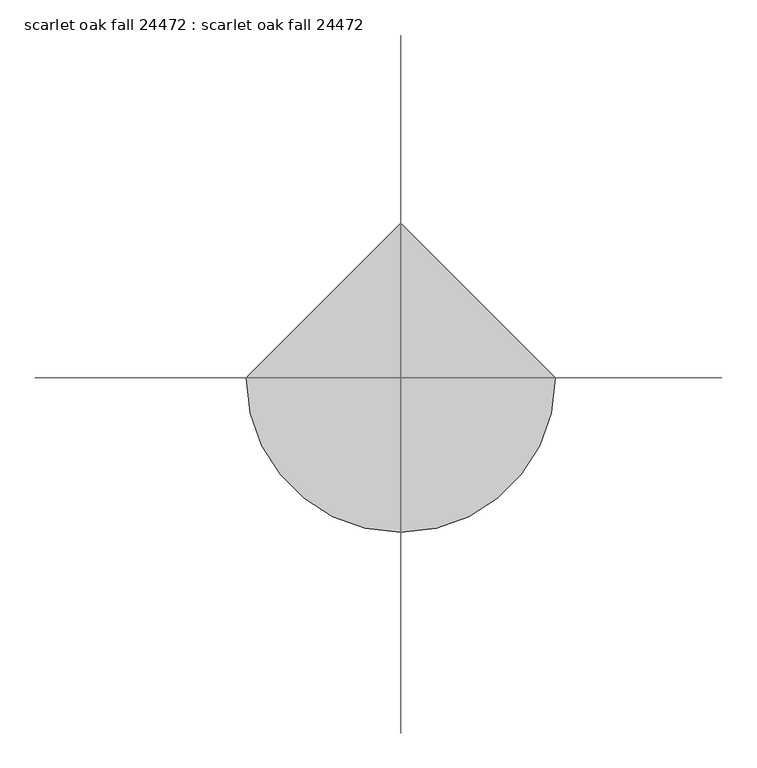
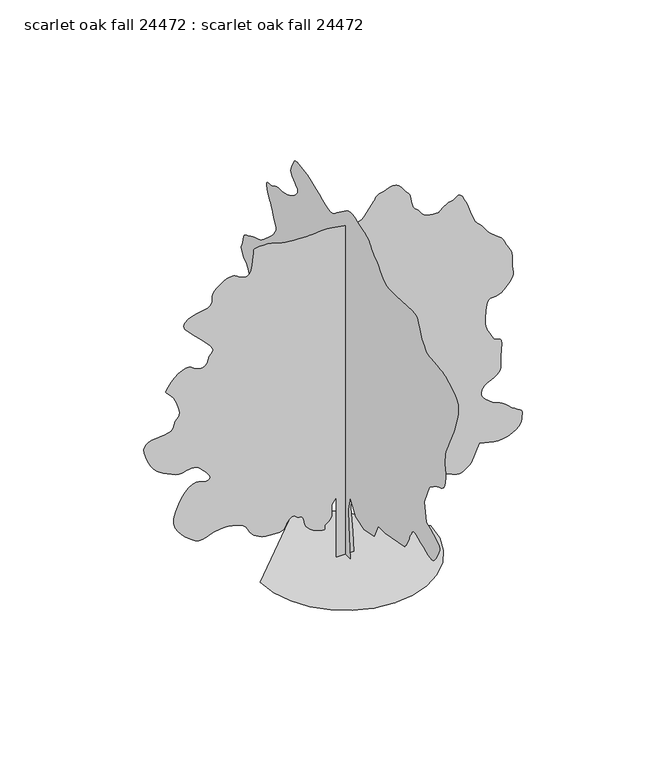
"""IFC4 building model written with IfcOpenShell, lengths in millimetres: proxy geometry, scarlet oak fall 24472 : scarlet oak fall 24472."""

import ifcopenshell
import ifcopenshell.guid

model = None  # the IFC model being written
_history = None  # IfcOwnerHistory: only IFC2X3 demands one
_inside = {}  # id of a spatial element -> (the spatial element, [elements in it])
_under = {}  # id of a project, library or spatial element -> (it, [spatial elements below it])
_declared = {}  # id of a project -> (the project, [libraries it declares])
_typed = {}  # id of a type object -> (the type object, [elements of that type])
_made_of = {}  # id of a material, layer set ... -> (it, [elements and type objects made of it])


def new_model(schema):
    """Start an empty IFC model of exactly this schema.

    Asked for "IFC4X3", IfcOpenShell would pick the latest addendum, in which some entities
    have other attributes; the version numbers below select the first issue.
    IFC2X3 requires an IfcOwnerHistory on every rooted entity: one is made here for all.
    """
    global model, _history
    if schema == "IFC4X3":
        model = ifcopenshell.file(schema_version=(4, 3, 0, 0))
    else:
        model = ifcopenshell.file(schema=schema)
    _inside.clear()
    _under.clear()
    _declared.clear()
    _typed.clear()
    _made_of.clear()
    _history = None
    if model.schema == "IFC2X3":
        org = make("IfcOrganization", Name="unknown")
        user = make(
            "IfcPersonAndOrganization",
            ThePerson=make("IfcPerson", FamilyName="unknown"),
            TheOrganization=org,
        )
        app = make(
            "IfcApplication",
            ApplicationDeveloper=org,
            Version="unknown",
            ApplicationFullName="unknown",
            ApplicationIdentifier="unknown",
        )
        _history = make(
            "IfcOwnerHistory",
            OwningUser=user,
            OwningApplication=app,
            ChangeAction="ADDED",
            CreationDate=0,
        )
    return model


def make(cls, **values):
    """One entity of the class cls with the attributes given. An attribute that is None is left unset."""
    return model.create_entity(
        cls, **{name: value for name, value in values.items() if value is not None}
    )


def rooted(cls, **values):
    """An entity with a GlobalId (a new one), such as an element, a storey or a relation."""
    return make(cls, GlobalId=ifcopenshell.guid.new(), OwnerHistory=_history, **values)


def si_unit(unit_type, name, prefix=None):
    """IfcSIUnit, for example si_unit("LENGTHUNIT", "METRE", prefix="MILLI")."""
    return make("IfcSIUnit", UnitType=unit_type, Prefix=prefix, Name=name)


def assignment(units):
    """IfcUnitAssignment: the units of a project."""
    return None if units is None else make("IfcUnitAssignment", Units=units)


def point(xyz):
    """IfcCartesianPoint."""
    return None if xyz is None else make("IfcCartesianPoint", Coordinates=xyz)


def direction(xyz):
    """IfcDirection."""
    return None if xyz is None else make("IfcDirection", DirectionRatios=xyz)


def frame(location, z_axis=None, x_axis=None):
    """IfcAxis2Placement3D, a coordinate frame: its origin and axes. An axis left out is left unset."""
    return make(
        "IfcAxis2Placement3D",
        Location=point(location),
        Axis=direction(z_axis),
        RefDirection=direction(x_axis),
    )


def origin():
    """The frame at (0, 0, 0) with its axes left unset."""
    return frame((0.0, 0.0, 0.0))


def place(relative_to, where):
    """IfcLocalPlacement: puts the frame where relative to a parent placement (None: the world)."""
    return make(
        "IfcLocalPlacement", PlacementRelTo=relative_to, RelativePlacement=where
    )


def context(
    kind, dimensions, precision=None, world=None, true_north=None, identifier=None
):
    """IfcGeometricRepresentationContext, for example the 3D "Model" context."""
    return make(
        "IfcGeometricRepresentationContext",
        ContextIdentifier=identifier,
        ContextType=kind,
        CoordinateSpaceDimension=dimensions,
        Precision=precision,
        WorldCoordinateSystem=world,
        TrueNorth=true_north,
    )


def project(units=None, contexts=None):
    """IfcProject with its units and contexts."""
    return rooted(
        "IfcProject",
        Name="project",
        RepresentationContexts=contexts,
        UnitsInContext=assignment(units),
    )


def spatial(cls, under=None, at=None, **own):
    """A site, building, storey or space (cls), placed at a placement, below another one or the project."""
    s = rooted(cls, ObjectPlacement=at, **own)
    if under is not None:
        _under.setdefault(under.id(), (under, []))[1].append(s)
    return s


def point_list(points):
    """IfcCartesianPointList2D or 3D."""
    cls = (
        "IfcCartesianPointList2D" if len(points[0]) == 2 else "IfcCartesianPointList3D"
    )
    return make(cls, CoordList=points)


def triangles(points, corners, closed=None, point_numbers=None):
    """IfcTriangulatedFaceSet: each triangle names its three corners, points numbered from 1."""
    return make(
        "IfcTriangulatedFaceSet",
        Coordinates=point_list(points),
        Closed=closed,
        CoordIndex=corners,
        PnIndex=point_numbers,
    )


def shape(context_of_items, identifier, shape_type, items):
    """IfcShapeRepresentation: the items that make up one representation, for example the "Body"."""
    return make(
        "IfcShapeRepresentation",
        ContextOfItems=context_of_items,
        RepresentationIdentifier=identifier,
        RepresentationType=shape_type,
        Items=items,
    )


def source(mapping_origin, context_of_items, identifier, shape_type, items):
    """IfcRepresentationMap: a shape defined once, which mapped items show again and again."""
    return make(
        "IfcRepresentationMap",
        MappingOrigin=mapping_origin,
        MappedRepresentation=shape(context_of_items, identifier, shape_type, items),
    )


def transform(
    local_origin,
    x_axis=None,
    y_axis=None,
    z_axis=None,
    scale=None,
    scale2=None,
    scale3=None,
    uniform=True,
):
    """IfcCartesianTransformationOperator3D, or its non-uniform kind. x_axis, y_axis, z_axis: its Axis1, 2, 3."""
    if uniform:
        return make(
            "IfcCartesianTransformationOperator3D",
            Axis1=direction(x_axis),
            Axis2=direction(y_axis),
            LocalOrigin=point(local_origin),
            Scale=scale,
            Axis3=direction(z_axis),
        )
    return make(
        "IfcCartesianTransformationOperator3DnonUniform",
        Axis1=direction(x_axis),
        Axis2=direction(y_axis),
        LocalOrigin=point(local_origin),
        Scale=scale,
        Axis3=direction(z_axis),
        Scale2=scale2,
        Scale3=scale3,
    )


def mapped(mapping_source, mapping_target):
    """IfcMappedItem: shows the shape of a source again, moved by a transform."""
    return make(
        "IfcMappedItem", MappingSource=mapping_source, MappingTarget=mapping_target
    )


def made_of(thing, what):
    """Note that an element or type object is made of a material, layer set ...; save() writes the relation."""
    if what is not None:
        _made_of.setdefault(what.id(), (what, []))[1].append(thing)
    return thing


def element(
    cls,
    number,
    at=None,
    inside=None,
    cuts=None,
    type_object=None,
    material=None,
    context=None,
    identifier="Body",
    shape_type=None,
    held_by="IfcProductDefinitionShape",
    body=None,
    shapes=None,
    **own,
):
    """One element of the class cls, such as IfcWall. Its Tag is "e" and its number.

    at: its placement. inside: the storey or other place that contains it. cuts: it is an
    opening in that element (IfcRelVoidsElement). A single representation is given by context,
    identifier, shape_type and body (its items); several are given by shapes. held_by: the class
    of the entity that holds the representations. save() writes the other relations.
    """
    e = rooted(cls, Tag="e%d" % number, ObjectPlacement=at, **own)
    if body is not None:
        shapes = [shape(context, identifier, shape_type, body)]
    if shapes is not None:
        e.Representation = make(held_by, Representations=shapes)
    if inside is not None:
        _inside.setdefault(inside.id(), (inside, []))[1].append(e)
    if cuts is not None:
        rooted(
            "IfcRelVoidsElement", RelatingBuildingElement=cuts, RelatedOpeningElement=e
        )
    if type_object is not None:
        _typed.setdefault(type_object.id(), (type_object, []))[1].append(e)
    return made_of(e, material)


def aggregate(whole, parts):
    """IfcRelAggregates: a whole, such as a stair, and the parts it consists of."""
    return rooted("IfcRelAggregates", RelatingObject=whole, RelatedObjects=parts)


def save(model, path):
    """Write the relations noted so far, then the file.

    IfcRelAggregates (storeys below a building ...), IfcRelContainedInSpatialStructure (elements
    in a storey), IfcRelDefinesByType, IfcRelAssociatesMaterial and IfcRelDeclares: one each for
    every whole, place, type object, material and project.
    """
    for whole, parts in _under.values():
        aggregate(whole, parts)
    for where, things in _inside.values():
        rooted(
            "IfcRelContainedInSpatialStructure",
            RelatedElements=things,
            RelatingStructure=where,
        )
    for kind, things in _typed.values():
        rooted("IfcRelDefinesByType", RelatedObjects=things, RelatingType=kind)
    for what, things in _made_of.values():
        rooted("IfcRelAssociatesMaterial", RelatedObjects=things, RelatingMaterial=what)
    for by, libraries in _declared.values():
        rooted("IfcRelDeclares", RelatingContext=by, RelatedDefinitions=libraries)
    model.write(path)


def scarlet_oak_fall_24472_scarlet_oak_fall_24472_7ddbc09d(model_context):
    return source(origin(), model_context, "Body", "Tessellation", [
        triangles([(0.0175265, 310.9036245, 0.0), (0.0175265, -298.2620451, 0.0), (0.0175265, -200.0097575, 1159.3779247), (0.0175265, -180.3587949, 1709.5902706), (0.0175265, -298.2620451, 2220.5035618), (0.0175265, -612.6708881, 1709.5902706), (0.0175265, -1123.5817085, 1552.3870754), (0.0175265, -1713.0954346, 1689.9407433), (0.0175265, -1948.9013901, 2181.2021816), (0.0175265, -2361.5625389, 2181.2021816), (0.0175265, -3501.2886108, 2397.3587551), (0.0175265, -3543.2238419, 2447.9453476), (0.0175265, -3584.1434372, 2498.8747971), (0.0175265, -3622.9800201, 2550.4902512), (0.0175265, -3658.7176643, 2603.1445953), (0.0175265, -3690.3407341, 2657.1703674), (0.0175265, -3716.8074326, 2712.9233597), (0.0175265, -3737.102124, 2770.7082047), (0.0175265, -3756.8125488, 2830.2458496), (0.0175265, -3781.6790543, 2890.7994209), (0.0175265, -3810.8383209, 2952.2166023), (0.0175265, -3843.4264481, 3014.3197884), (0.0175265, -3878.6054054, 3076.9307922), (0.0175265, -3915.4862938, 3139.8972977), (0.0175265, -3953.2560814, 3203.0164101), (0.0175265, -3971.239286, 3223.4125488), (0.0175265, -3996.1057915, 3239.8717186), (0.0175265, -4034.7139, 3248.4060814), (0.0175265, -4093.9466217, 3245.0786682), (0.0175265, -4180.6878387, 3225.9525101), (0.0175265, -4301.7949814, 3187.039769), (0.0175265, -4464.1516411, 3124.4287651), (0.0175265, -4635.5763519, 3050.7434372), (0.0175265, -4781.5502907, 2984.9826256), (0.0175265, -4905.5273163, 2932.6079155), (0.0175265, -5010.9377426, 2899.1561783), (0.0175265, -5101.2345566, 2890.113707), (0.0175265, -5179.8222015, 2910.9670853), (0.0175265, -5250.1801163, 2967.228186), (0.0175265, -5321.172876, 3055.8486488), (0.0175265, -5394.553862, 3163.7225876), (0.0175265, -5463.1339783, 3281.2229736), (0.0175265, -5519.6741318, 3398.7233597), (0.0175265, -5556.9613907, 3506.5970078), (0.0175265, -5567.8072403, 3595.2430504), (0.0175265, -5544.9470078, 3654.9838806), (0.0175265, -5489.0922775, 3699.9671814), (0.0175265, -5408.4727798, 3750.0815643), (0.0175265, -5307.2539581, 3804.513707), (0.0175265, -5189.4995178, 3862.3750008), (0.0175265, -5059.4004822, 3922.8268341), (0.0175265, -4921.0467178, 3984.9805984), (0.0175265, -4778.5783791, 4047.9982635), (0.0175265, -4660.6716225, 4716.1196915), (0.0175265, -4955.4132248, 5403.875386), (0.0175265, -4964.7097504, 5417.0071426), (0.0175265, -4979.1367767, 5433.0346527), (0.0175265, -5003.9015442, 5454.9298279), (0.0175265, -5044.1101364, 5485.5872589), (0.0175265, -5104.9430511, 5527.903862), (0.0175265, -5191.5825302, 5584.850386), (0.0175265, -5309.1334946, 5659.3487457), (0.0175265, -5436.6669891, 5726.8364868), (0.0175265, -5549.7478775, 5770.9308884), (0.0175265, -5648.4011581, 5806.7955597), (0.0175265, -5732.6279938, 5849.5441132), (0.0175265, -5802.4016418, 5914.2884171), (0.0175265, -5857.7482635, 6016.1426651), (0.0175265, -5898.6422791, 6170.2443054), (0.0175265, -5922.3152527, 6321.6030899), (0.0175265, -5929.1223953, 6418.6564682), (0.0175265, -5923.915155, 6481.6735519), (0.0175265, -5911.4694031, 6530.949614), (0.0175265, -5896.6354248, 6586.7537659), (0.0175265, -5884.2152527, 6669.354538), (0.0175265, -5879.0080124, 6799.0722015), (0.0175265, -5880.8369705, 6942.175676), (0.0175265, -5888.8632248, 7060.8701752), (0.0175265, -5906.8464294, 7169.2769302), (0.0175265, -5938.5712372, 7281.4433395), (0.0175265, -5987.8467178, 7411.4917969), (0.0175265, -6058.4336884, 7573.5179535), (0.0175265, -6154.0900589, 7781.5947876), (0.0175265, -6244.9205612, 7969.6821442), (0.0175265, -6305.4738419, 8083.1694031), (0.0175265, -6346.419017, 8153.3494217), (0.0175265, -6378.4484573, 8211.4900589), (0.0175265, -6412.2045364, 8288.8835907), (0.0175265, -6458.3057922, 8416.8234558), (0.0175265, -6527.4701752, 8626.5513519), (0.0175265, -6601.9935333, 8869.1720078), (0.0175265, -6652.1329147, 9078.1127426), (0.0175265, -6670.2940155, 9258.1732635), (0.0175265, -6648.9075302, 9414.1800201), (0.0175265, -6580.4541504, 9550.9338821), (0.0175265, -6457.3407349, 9673.2345566), (0.0175265, -6271.9968155, 9785.9340729), (0.0175265, -6092.164769, 9878.5679535), (0.0175265, -5973.8772217, 9942.3477814), (0.0175265, -5892.0130325, 9984.43591), (0.0175265, -5821.4772217, 10012.1214294), (0.0175265, -5737.1998077, 10032.5690186), (0.0175265, -5614.0858109, 10053.0154449), (0.0175265, -5427.0402512, 10080.7009644), (0.0175265, -5226.405986, 10102.5205627), (0.0175265, -5070.8056, 10110.9526062), (0.0175265, -4947.513707, 10121.4182465), (0.0175265, -4843.8310822, 10149.4339783), (0.0175265, -4747.0061783, 10210.4442078), (0.0175265, -4644.3394798, 10319.9445007), (0.0175265, -4523.1050194, 10493.3501953), (0.0175265, -4417.2379349, 10684.0025116), (0.0175265, -4354.6778, 10837.2152527), (0.0175265, -4313.7837845, 10956.3661194), (0.0175265, -4272.8641891, 11044.9362946), (0.0175265, -4210.3040543, 11106.353476), (0.0175265, -4104.4369698, 11144.0476868), (0.0175265, -3933.5965256, 11161.4710419), (0.0175265, -2990.3674713, 11102.5176636), (0.0175265, -2816.5045372, 11105.5663147), (0.0175265, -2674.9503868, 11105.1593628), (0.0175265, -2554.6812744, 11112.322879), (0.0175265, -2444.7449615, 11138.027124), (0.0175265, -2334.1178478, 11193.3225861), (0.0175265, -2211.8040928, 11289.1574341), (0.0175265, -2066.8032051, 11436.5786682), (0.0175265, -1927.0752514, 11585.474231), (0.0175265, -1822.4043148, 11686.9215271), (0.0175265, -1744.5483112, 11753.6721039), (0.0175265, -1685.2519306, 11798.4275116), (0.0175265, -1636.2706181, 11833.8858124), (0.0175265, -1589.3492088, 11872.7729736), (0.0175265, -1536.2428574, 11927.8405426), (0.0175265, -1485.2548359, 11992.8644806), (0.0175265, -1443.5456085, 12053.4177612), (0.0175265, -1401.1529926, 12109.8573395), (0.0175265, -1348.1024517, 12162.4855225), (0.0175265, -1274.4272976, 12211.7104248), (0.0175265, -1170.1577173, 12257.8366791), (0.0175265, -1025.3294209, 12301.1944977), (0.0175265, -862.7415253, 12348.971814), (0.0175265, -711.1517956, 12401.9057922), (0.0175265, -569.5289721, 12450.7249054), (0.0175265, -436.8469909, 12486.1320465), (0.0175265, -312.0695054, 12498.8580139), (0.0175265, -194.1657283, 12479.604538), (0.0175265, -82.1065163, 12419.1012543), (0.0175265, 507.4081999, 11986.7939209), (0.0175265, 571.2282506, 11928.7044434), (0.0175265, 632.9883253, 11875.7704651), (0.0175265, 700.2449759, 11833.124231), (0.0175265, 780.5673986, 11805.9712372), (0.0175265, 881.5121092, 11799.4437286), (0.0175265, 1010.6431807, 11818.6960419), (0.0175265, 1175.5247589, 11868.8871643), (0.0175265, 1362.6338322, 11943.4105225), (0.0175265, 1551.1170948, 12027.2309875), (0.0175265, 1737.537838, 12112.7780914), (0.0175265, 1918.4594982, 12192.4581116), (0.0175265, 2090.445512, 12258.7517395), (0.0175265, 2250.0539383, 12304.0652527), (0.0175265, 2393.8535912, 12320.8549255), (0.0175265, 2524.6458984, 12330.0241333), (0.0175265, 2646.1466217, 12350.8775116), (0.0175265, 2756.3317566, 12373.4331116), (0.0175265, 2853.0805023, 12387.7578186), (0.0175265, 2934.3860046, 12383.8720093), (0.0175265, 2998.139962, 12351.7914093), (0.0175265, 3042.3105217, 12281.5352325), (0.0175265, 3081.7819496, 12193.2708527), (0.0175265, 3127.0957535, 12111.863031), (0.0175265, 3169.6661201, 12034.5712372), (0.0175265, 3200.9081085, 11958.6502899), (0.0175265, 3212.1856178, 11881.3840759), (0.0175265, 3194.9389961, 11799.9762543), (0.0175265, 3140.5830116, 11711.6862946), (0.0175265, 3057.3979729, 11630.7877441), (0.0175265, 2968.3455597, 11567.4148682), (0.0175265, 2886.8880318, 11512.6519318), (0.0175265, 2826.3850388, 11457.5343658), (0.0175265, 2800.2738419, 11393.1452728), (0.0175265, 2821.9146721, 11310.5445007), (0.0175265, 2904.7694984, 11200.765155), (0.0175265, 3019.1712364, 11091.3927612), (0.0175265, 3127.0448845, 11011.6115845), (0.0175265, 3229.076738, 10954.8173767), (0.0175265, 3325.9522202, 10914.5582062), (0.0175265, 3418.3576263, 10884.2309875), (0.0175265, 3507.0033783, 10857.3826263), (0.0175265, 3592.525193, 10827.4112), (0.0175265, 3677.9455605, 10804.3219116), (0.0175265, 3765.7785713, 10796.7026093), (0.0175265, 3855.9995178, 10795.9654449), (0.0175265, 3948.6333984, 10793.5016418), (0.0175265, 4043.6802132, 10780.7256775), (0.0175265, 4141.139962, 10749.0264496), (0.0175265, 4240.9873558, 10689.8695953), (0.0175265, 4344.1874519, 10637.3169891), (0.0175265, 4445.6350388, 10618.4704651), (0.0175265, 4536.4402519, 10614.0509674), (0.0175265, 4607.6617767, 10604.8306), (0.0175265, 4650.3338814, 10571.5570496), (0.0175265, 4655.540831, 10494.9500977), (0.0175265, 4614.3674721, 10355.8085907), (0.0175265, 4553.5089775, 10209.3779938), (0.0175265, 4502.988224, 10110.7247131), (0.0175265, 4458.6400589, 10040.2394806), (0.0175265, 4416.3743248, 9978.3653503), (0.0175265, 4372.025869, 9905.4918915), (0.0175265, 4321.4798264, 9802.0377411), (0.0175265, 4260.6469116, 9648.393631), (0.0175265, 4196.3595566, 9497.2633209), (0.0175265, 4141.038224, 9401.8104263), (0.0175265, 4098.7472008, 9343.1361008), (0.0175265, 4073.6522209, 9302.3438232), (0.0175265, 4069.8675682, 9260.5353287), (0.0175265, 4091.5336876, 9198.7629364), (0.0175265, 4142.740155, 9098.1789597), (0.0175265, 4233.9008698, 8964.8539581), (0.0175265, 4361.815155, 8823.2998077), (0.0175265, 4510.3796333, 8682.0758698), (0.0175265, 4663.3894798, 8549.7926651), (0.0175265, 4804.7404449, 8435.0357162), (0.0175265, 4918.2277039, 8346.4149628), (0.0175265, 4987.7217178, 8292.4909286), (0.0175265, 5049.4185333, 8258.7592667), (0.0175265, 5142.0524139, 8224.6723938), (0.0175265, 5253.2537659, 8189.9000977), (0.0175265, 5370.6524139, 8154.0860046), (0.0175265, 5481.8537659, 8116.9004837), (0.0175265, 5574.4876465, 8078.0133224), (0.0175265, 5636.1838806, 8037.0425674), (0.0175265, 5687.8475876, 8003.0068542), (0.0175265, 5753.6336884, 7978.9530899), (0.0175265, 5825.9217178, 7955.5853302), (0.0175265, 5897.1941116, 7923.6064682), (0.0175265, 5959.8815643, 7873.7717194), (0.0175265, 6006.3891907, 7796.7589783), (0.0175265, 6029.1982635, 7683.3222977), (0.0175265, 6047.8674728, 7569.3780899), (0.0175265, 6079.9474915, 7488.7835907), (0.0175265, 6114.7709473, 7429.1447891), (0.0175265, 6141.7204651, 7378.0903473), (0.0175265, 6150.0769318, 7323.2774139), (0.0175265, 6129.2235535, 7252.2846542), (0.0175265, 6068.4917953, 7152.7674728), (0.0175265, 5993.1045364, 7059.5493256), (0.0175265, 5932.1448853, 7003.8213318), (0.0175265, 5880.8113907, 6967.6776077), (0.0175265, 5834.2787659, 6933.2349426), (0.0175265, 5787.7711395, 6882.638031), (0.0175265, 5736.437645, 6798.030986), (0.0175265, 5675.4779938, 6661.5055984), (0.0175265, 5609.0314682, 6524.7523178), (0.0175265, 5548.0712357, 6438.5447891), (0.0175265, 5498.1097504, 6383.604538), (0.0175265, 5464.6577225, 6340.6786697), (0.0175265, 5453.2026077, 6290.5642868), (0.0175265, 5469.2295364, 6213.9579163), (0.0175265, 5518.277124, 6091.6566605), (0.0175265, 5583.4283798, 5957.8747101), (0.0175265, 5644.7694031, 5854.0141891), (0.0175265, 5703.392569, 5771.4645767), (0.0175265, 5760.2629349, 5701.6141891), (0.0175265, 5816.4734573, 5635.9048279), (0.0175265, 5873.0136108, 5565.7242279), (0.0175265, 5930.9257736, 5482.4886108), (0.0175265, 5998.1338806, 5400.3959473), (0.0175265, 6076.3407349, 5333.4157333), (0.0175265, 6157.2904449, 5272.6339783), (0.0175265, 6232.753862, 5209.0832062), (0.0175265, 6294.4506775, 5133.8738434), (0.0175265, 6334.1505798, 5038.0139969), (0.0175265, 6343.5994217, 4912.614093), (0.0175265, 6351.5495178, 4814.1384178), (0.0175265, 6380.8355209, 4781.651738), (0.0175265, 6414.2369705, 4780.1024139), (0.0175265, 6434.5822403, 4774.4382248), (0.0175265, 6424.6508698, 4729.5816605), (0.0175265, 6367.3229736, 4610.4810814), (0.0175265, 6245.3519302, 4382.0589775), (0.0175265, 6117.819017, 4125.8490349), (0.0175265, 6040.8312744, 3937.3811783), (0.0175265, 5992.6981659, 3802.5071434), (0.0175265, 5951.8041504, 3707.1809853), (0.0175265, 5896.4575287, 3637.2800194), (0.0175265, 5805.0177612, 3578.7330116), (0.0175265, 5655.8437271, 3517.4428574), (0.0175265, 5483.6059845, 3467.7098465), (0.0175265, 5332.0187256, 3446.8561775), (0.0175265, 5192.8016418, 3445.2559845), (0.0175265, 5057.7244217, 3453.2825294), (0.0175265, 4918.5067566, 3461.2834946), (0.0175265, 4766.9197884, 3459.6833015), (0.0175265, 4594.7076256, 3438.8299232), (0.0175265, 4422.952993, 3420.1610046), (0.0175265, 4274.5661201, 3424.1741318), (0.0175265, 4144.0610046, 3439.8714294), (0.0175265, 4025.9254829, 3456.2544411), (0.0175265, 3914.6735527, 3462.3250008), (0.0175265, 3804.7930504, 3447.0849426), (0.0175265, 3690.7723938, 3399.5361008), (0.0175265, 3581.6540543, 3348.9900581), (0.0175265, 3491.4078186, 3322.5233597), (0.0175265, 3422.1419884, 3305.6831085), (0.0175265, 3375.9139961, 3284.0422783), (0.0175265, 3354.7812744, 3243.1229736), (0.0175265, 3360.8009651, 3168.5484558), (0.0175265, 3396.0307915, 3045.815831), (0.0175265, 3452.8505791, 2915.4374519), (0.0175265, 3521.0243248, 2823.1846527), (0.0175265, 3598.6722015, 2762.7581085), (0.0175265, 3683.8638039, 2727.7567566), (0.0175265, 3774.7195953, 2711.8309845), (0.0175265, 3869.3600395, 2708.6053093), (0.0175265, 3965.8800201, 2711.7548264), (0.0175265, 4339.2598457, 2299.1064674), (0.0175265, 4368.5208504, 2252.6422977), (0.0175265, 4396.5877419, 2205.3220757), (0.0175265, 4422.2672791, 2156.2823364), (0.0175265, 4444.3144798, 2104.6617954), (0.0175265, 4461.5608109, 2049.6073071), (0.0175265, 4472.7877419, 1990.2551159), (0.0175265, 4476.800869, 1925.7468441), (0.0175265, 4476.115155, 1858.4875774), (0.0175265, 4471.314576, 1791.9167862), (0.0175265, 4458.2333977, 1726.7225098), (0.0175265, 4432.8082054, 1663.588282), (0.0175265, 4390.8726837, 1603.2049038), (0.0175265, 4328.3125488, 1546.2580891), (0.0175265, 4240.9873558, 1493.4361679), (0.0175265, 4157.7008698, 1448.5772781), (0.0175265, 4099.153862, 1413.687838), (0.0175265, 4049.1917953, 1386.7054733), (0.0175265, 3991.6610046, 1365.5650486), (0.0175265, 3910.4316605, 1348.2066605), (0.0175265, 3789.3245178, 1332.5653187), (0.0175265, 3612.1850395, 1316.5811199), (0.0175265, 3410.6865829, 1318.8721138), (0.0175265, 3225.0127419, 1354.1629829), (0.0175265, 3051.7084946, 1414.5488319), (0.0175265, 2887.3449806, 1492.1179344), (0.0175265, 2728.4933395, 1578.9707726), (0.0175265, 2571.6738419, 1667.1976547), (0.0175265, 2413.5029732, 1748.8916508), (0.0175265, 2272.4543152, 1823.1968536), (0.0175265, 2163.3739094, 1893.3770176), (0.0175265, 2077.3237839, 1957.7152416), (0.0175265, 2005.3681469, 2014.4892471), (0.0175265, 1938.5687359, 2061.9822784), (0.0175265, 1867.9871429, 2098.4769985), (0.0175265, 1784.687867, 2122.2512741), (0.0175265, 1693.0802319, 2142.3020851), (0.0175265, 1602.8492569, 2167.1661198), (0.0175265, 1512.9611389, 2194.438147), (0.0175265, 1422.387307, 2221.7075581), (0.0175265, 1330.0913418, 2246.5715927), (0.0175265, 1235.0471432, 2266.6224037), (0.0175265, 1136.2233061, 2279.4544693), (0.0175265, 1035.1643583, 2286.1575485), (0.0175265, 934.1027945, 2289.7669212), (0.0175265, 833.0438467, 2290.7981083), (0.0175265, 731.9848263, 2289.7669212), (0.0175265, 630.9258785, 2287.1887356), (0.0175265, 529.864351, 2283.5795082), (0.0175265, 428.8053669, 2279.4544693), (0.0175265, 232.3013002, 1984.6976063), (0.0175265, 192.9998656, 1532.7376934), (284.9321357, 0.0006104, 0.0093596), (-304.5815722, 0.0006104, 0.0093596), (-304.5815722, 0.0004832, 2161.5603573), (-461.7872563, 0.0004832, 1945.4063999), (-461.7872563, 0.0005087, 1709.6004444), (-458.17792, 0.0005087, 1654.888813), (-458.17792, 0.0005087, 1600.3473747), (-465.3965927, 0.0005087, 1546.1514095), (-483.4407675, 0.0005341, 1492.4709652), (-515.9248312, 0.0005341, 1439.4789963), (-566.4555768, 0.0005341, 1387.3429344), (-638.6398699, 0.0005341, 1336.2406757), (-695.1853283, 0.0005341, 1283.1902802), (-710.8266701, 0.0005341, 1229.4514091), (-707.2172974, 0.0005341, 1181.559783), (-706.0133738, 0.0005341, 1146.037896), (-728.8733156, 0.0005341, 1129.4237211), (-797.4482723, 0.0005341, 1138.2476738), (-933.3966602, 0.0005341, 1179.0375532), (-1088.4814528, 0.0005341, 1242.5731373), (-1204.3791023, 0.0005341, 1314.3561104), (-1287.6199516, 0.0005341, 1393.0172974), (-1344.7395756, 0.0005341, 1477.1750965), (-1382.2654827, 0.0005087, 1565.4579346), (-1406.7282337, 0.0005087, 1656.4914768), (-1424.6607147, 0.0005087, 1748.9018246), (-1429.2428478, 0.0005087, 1774.0502895), (-1436.0601643, 0.0005087, 1798.5130405), (-1447.3453766, 0.0005087, 1821.6042183), (-1465.3361389, 0.0005087, 1842.6277897), (-1492.2602222, 0.0005087, 1860.9031277), (-1530.3602222, 0.0005087, 1875.7417568), (-1581.8637646, 0.0005087, 1886.4554924), (-1633.3673069, 0.0005087, 1904.0983109), (-1673.8702126, 0.0005087, 1933.7757145), (-1709.219363, 0.0004832, 1965.8584946), (-1745.2543728, 0.0004832, 1990.7225292), (-1787.8222687, 0.0004832, 1998.7438419), (-1842.7623745, 0.0004832, 1980.2958401), (-1915.9220078, 0.0005087, 1925.7544018), (-1980.257761, 0.0005087, 1849.4451061), (-2016.7524811, 0.0005087, 1774.8530022), (-2043.2776062, 0.0005087, 1706.1053089), (-2077.707336, 0.0005087, 1647.3247398), (-2137.9206665, 0.0005087, 1602.6409847), (-2241.7862743, 0.0005087, 1576.1716702), (-2407.1834461, 0.0005087, 1572.0466312), (-2589.9363899, 0.0005087, 1584.1929829), (-2738.3232628, 0.0005087, 1604.2437939), (-2858.8464294, 0.0005087, 1632.8898651), (-2958.0839767, 0.0005087, 1670.8145851), (-3042.5389961, 0.0005087, 1718.7089001), (-3118.713707, 0.0005087, 1777.2608494), (-3193.211776, 0.0005087, 1847.1541122), (-3256.3817574, 0.0005087, 1923.8062649), (-3301.7205597, 0.0004832, 2000.8063614), (-3340.1507721, 0.0004832, 2076.0843246), (-3382.7214294, 0.0004832, 2147.5827221), (-3440.4048271, 0.0004832, 2213.2367088), (-3524.2247108, 0.0004832, 2270.9860909), (-3645.154248, 0.0004832, 2318.7660233), (-3766.7439194, 0.0004832, 2355.0854633), (-3854.9580116, 0.0004578, 2380.7522106), (-3924.6302124, 0.0004578, 2397.1378384), (-3990.5180511, 0.0004578, 2405.6162453), (-4067.3781853, 0.0004578, 2407.5645275), (-4170.0451744, 0.0004578, 2404.3564384), (-4313.275676, 0.0004578, 2397.3663128), (-4470.7555984, 0.0004578, 2372.5607048), (-4610.7351357, 0.0004832, 2326.4420082), (-4739.6909271, 0.0004832, 2276.1982727), (-4864.1763519, 0.0004832, 2239.0176933), (-4990.7447891, 0.0004832, 2232.0859943), (-5125.8725876, 0.0004832, 2272.5889), (-5276.1389969, 0.0004578, 2377.7169308), (-5433.3648651, 0.0004578, 2518.3058784), (-5578.5257721, 0.0004578, 2657.8560814), (-5702.0461395, 0.0004324, 2802.5853287), (-5794.2736496, 0.0004324, 2958.6429543), (-5845.6071442, 0.0004324, 3132.226545), (-5846.4198853, 0.0004069, 3329.5336876), (-5787.0601364, 0.0004069, 3556.7366798), (-5687.7208511, 0.0003815, 3785.8956573), (-5577.0276077, 0.0003815, 3982.4153481), (-5458.1046341, 0.0003561, 4142.4861008), (-5334.0255798, 0.0003561, 4262.3232628), (-5207.8635132, 0.0003561, 4338.1677612), (-5082.7432434, 0.0003561, 4366.2602325), (-4961.7378387, 0.0003561, 4342.765155), (-4847.6154442, 0.0003561, 4303.2428581), (-4746.5742279, 0.0003561, 4286.3770271), (-4666.8183403, 0.0003561, 4293.2606186), (-4616.6277992, 0.0003561, 4324.8833977), (-4604.2582054, 0.0003561, 4382.2874519), (-4637.9384171, 0.0003561, 4466.5139969), (-4725.9240349, 0.0003306, 4578.5786682), (-4828.540155, 0.0003306, 4690.9738426), (-4906.7470093, 0.0003306, 4777.5877419), (-4969.8146713, 0.0003306, 4841.5195953), (-5027.0414108, 0.0003306, 4885.8680511), (-5087.7220093, 0.0003306, 4913.7064682), (-5161.1024139, 0.0003052, 4928.1590744), (-5256.5047302, 0.0003052, 4932.2739395), (-5354.3458511, 0.0003306, 4923.0535721), (-5435.3717194, 0.0003306, 4901.7938232), (-5509.1584946, 0.0003306, 4878.1464294), (-5585.3584946, 0.0003306, 4861.6872597), (-5673.5728775, 0.0003306, 4862.0936302), (-5783.4533798, 0.0003306, 4888.9666992), (-5924.6261581, 0.0003052, 4951.9332047), (-6074.4356186, 0.0003052, 5027.2698853), (-6206.363031, 0.0003052, 5092.6240356), (-6324.2192093, 0.0003052, 5159.730986), (-6431.7376465, 0.0003052, 5240.2231659), (-6532.7529922, 0.0003052, 5345.7859085), (-6631.0004837, 0.0002798, 5488.1528), (-6730.2891907, 0.0002798, 5679.0085922), (-6812.3818542, 0.0002543, 5877.0523178), (-6857.6953674, 0.0002543, 6036.2594604), (-6867.9569504, 0.0002543, 6161.1006775), (-6844.8682434, 0.0002289, 6256.0204651), (-6790.157048, 0.0002289, 6325.5144791), (-6705.5494217, 0.0002289, 6374.0283783), (-6592.7225876, 0.0002289, 6406.0578186), (-6459.5249039, 0.0002289, 6424.4473938), (-6318.7834946, 0.0002289, 6435.2932434), (-6179.7187271, 0.0002289, 6447.8157349), (-6051.677124, 0.0002289, 6471.3613907), (-5943.9302124, 0.0002289, 6515.201738), (-5865.7239395, 0.0002289, 6588.5821426), (-5826.3536682, 0.0002035, 6700.8252914), (-5797.2705597, 0.0002035, 6809.207048), (-5752.3384186, 0.0002035, 6879.7934372), (-5704.6878387, 0.0002035, 6934.9115845), (-5667.3244217, 0.0002035, 6996.8874527), (-5653.3543442, 0.000178, 7088.0987457), (-5675.8082062, 0.000178, 7230.8720078), (-5747.7660233, 0.000178, 7447.5343643), (-5849.6708496, 0.0001526, 7660.9451752), (-5947.1305984, 0.0001526, 7795.2858124), (-6030.8237457, 0.0001526, 7874.990831), (-6091.5043442, 0.0001272, 7924.4192093), (-6119.8508698, 0.0001272, 7968.0055023), (-6106.6173752, 0.0001272, 8030.1848465), (-6042.5079163, 0.0001272, 8135.3156387), (-5939.1805023, 0.0001272, 8266.5064682), (-5819.6738434, 0.0001017, 8386.0137085), (-5691.911293, 0.0001017, 8486.9528961), (-5563.7941132, 0.0001017, 8562.4674728), (-5443.2712372, 0.0001017, 8605.6473953), (-5338.1910233, 0.0001017, 8609.6605225), (-5256.5047302, 0.0001017, 8567.6235535), (-5176.4183395, 0.0001017, 8504.9361008), (-5077.7650589, 0.0001017, 8456.015831), (-4970.8564682, 0.0001017, 8427.3646729), (-4866.0050194, 0.0001017, 8425.5357147), (-4773.5490349, 0.0001017, 8457.0570465), (-4703.7753868, 0.0001017, 8528.4311783), (-4666.9962364, 0.0001017, 8646.2111984), (-4633.2904449, 0.0001017, 8758.5043442), (-4580.3567574, 7.63e-05, 8825.0776062), (-4529.8360039, 7.63e-05, 8869.9853302), (-4503.3693054, 7.63e-05, 8917.3051163), (-4522.6224907, 7.63e-05, 8991.0924728), (-4609.2366806, 7.63e-05, 9115.425), (-4784.902993, 5.09e-05, 9314.3326263), (-5005.1718155, 5.09e-05, 9539.0212372), (-5202.0725876, 2.54e-05, 9728.3021255), (-5361.8639969, 2.54e-05, 9887.6871643), (-5470.753862, 2.54e-05, 10022.6626465), (-5515.0511581, 0.0, 10138.7404449), (-5480.9642853, 0.0, 10241.4074341), (-5354.7522217, 0.0, 10336.1493256), (-5186.4258682, 0.0, 10409.1483582), (-5035.6519318, 0.0, 10450.8562775), (-4903.089093, 0.0, 10473.3095581), (-4789.4242287, -2.54e-05, 10488.5493256), (-4695.3424713, -2.54e-05, 10508.5899628), (-4621.5554054, -2.54e-05, 10545.4958496), (-4568.7234558, -2.54e-05, 10611.2569519), (-4542.3837845, -2.54e-05, 10689.0568542), (-4538.3706573, -2.54e-05, 10757.2306), (-4542.9424713, -2.54e-05, 10820.603476), (-4542.3837845, -2.54e-05, 10883.9763519), (-4522.9018341, -5.09e-05, 10952.1500977), (-4470.7555984, -5.09e-05, 11029.95), (-4372.2290543, -5.09e-05, 11122.1780914), (-4251.6300201, -5.09e-05, 11213.4399628), (-4141.3431473, -5.09e-05, 11284.4333038), (-4039.6667953, -7.63e-05, 11334.0895752), (-3944.8487457, -7.63e-05, 11361.4204651), (-3855.1867767, -7.63e-05, 11365.3830139), (-3768.9536682, -7.63e-05, 11344.909845), (-3684.4733597, -5.09e-05, 11299.0382263), (-3597.3766411, -5.09e-05, 11242.9544403), (-3507.5623558, -5.09e-05, 11199.2408295), (-3419.4497108, -5.09e-05, 11177.8549255), (-3337.5093636, -5.09e-05, 11188.8019318), (-3266.2369698, -5.09e-05, 11242.0149628), (-3210.1028961, -7.63e-05, 11347.5015472), (-3173.5522202, -7.63e-05, 11515.1924744), (-3151.7337845, -7.63e-05, 11695.2524139), (-3136.0873558, -0.0001017, 11834.3939209), (-3125.5970078, -0.0001017, 11937.4666992), (-3119.2471046, -0.0001017, 12009.2472015), (-3115.9705605, -0.0001017, 12054.5607147), (-3114.776738, -0.0001017, 12078.2336884), (-3114.5988419, -0.0001017, 12085.0414124), (-3088.7669884, -0.0001017, 12089.0539581), (-3018.5869698, -0.0001017, 12097.8929535), (-2915.0563705, -0.0001017, 12106.7075317), (-2789.1995178, -0.0001017, 12110.7200775), (-2651.988707, -0.0001017, 12105.1064667), (-2514.4299522, -0.0001017, 12085.0414124), (-2387.5340641, -0.0001017, 12045.7472992), (-2271.1766315, -0.0001017, 12002.0336884), (-2154.476342, -0.0001017, 11970.3600403), (-2032.2769695, -0.0001017, 11948.286969), (-1899.419672, -0.0001017, 11933.4541534), (-1750.7534557, -0.0001017, 11923.4466248), (-1581.1170078, -0.0001017, 11915.8261597), (-1385.3567184, -0.0001017, 11908.2056946), (-1196.4162163, -0.0001017, 11907.1139008), (-1040.8158302, -0.0001017, 11916.3342682), (-903.7777559, -0.0001017, 11929.3392883), (-770.5217182, -0.0001017, 11939.6002899), (-626.2675146, -0.0001017, 11940.5653473), (-456.2297467, -0.0001017, 11925.7325317), (-245.6314641, -0.0001017, 11888.5464294), (-32.7413631, -0.0001017, 11844.3247101), (138.8999065, -0.0001017, 11813.8451752), (276.1665915, -0.0001017, 11798.8333008), (385.9352365, -0.0001017, 11800.9924713), (475.0790686, -0.0001017, 11822.1004852), (550.4713417, -0.0001017, 11863.8072418), (618.9904152, -0.0001017, 11927.8405426), (913.7472782, -0.0001272, 12301.1944977), (957.9762646, -0.0001272, 12358.7770294), (993.267061, -0.0001272, 12412.929538), (1025.1186052, -0.0001272, 12462.586972), (1059.035285, -0.0001272, 12506.7575317), (1100.5134218, -0.0001272, 12544.3994202), (1155.0548601, -0.0001272, 12574.4731659), (1228.1561394, -0.0001272, 12595.9625519), (1317.7570656, -0.0001526, 12620.5994202), (1415.6080696, -0.0001526, 12653.4927612), (1517.9269695, -0.0001526, 12683.6176666), (1620.9366703, -0.0001526, 12700.0003876), (1720.8500484, -0.0001526, 12691.6439209), (1813.8876835, -0.0001526, 12647.5245209), (1896.2726257, -0.0001272, 12556.6684387), (1969.4296429, -0.0001272, 12453.0363922), (2036.4018631, -0.0001272, 12372.4168945), (2095.8124809, -0.0001272, 12306.5802155), (2146.2848362, -0.0001272, 12247.2966248), (2186.4447395, -0.0001272, 12186.2852325), (2214.9181469, -0.0001017, 12115.2918915), (2230.3283981, -0.0001017, 12026.0880341), (2241.0421337, -0.0001017, 11933.6320496), (2255.8807629, -0.0001017, 11856.6437256), (2274.1561008, -0.0001017, 11792.534848), (2295.1796722, -7.63e-05, 11738.736969), (2318.2682339, -7.63e-05, 11692.6618744), (2342.7309849, -7.63e-05, 11651.7678589), (2367.882066, -7.63e-05, 11613.4388031), (2393.3175774, -7.63e-05, 11596.1921814), (2419.7868919, -7.63e-05, 11576.5329163), (2448.3162552, -7.63e-05, 11552.0727814), (2479.9416504, -7.63e-05, 11520.3991333), (2515.6897591, -7.63e-05, 11479.0981659), (2556.5863907, -7.63e-05, 11425.7583984), (2603.677993, -7.63e-05, 11357.9916046), (2673.4772209, -5.09e-05, 11293.5769318), (2772.1307922, -5.09e-05, 11249.4831116), (2885.2113899, -5.09e-05, 11221.8475891), (2998.2922783, -5.09e-05, 11206.9624512), (3096.9458496, -5.09e-05, 11200.9942108), (3166.7450775, -5.09e-05, 11200.2070496), (3193.211776, -5.09e-05, 11200.7907349), (3206.7754829, -5.09e-05, 11214.9387085), (3244.088031, -5.09e-05, 11251.4132263), (3299.9427612, -5.09e-05, 11301.3241333), (3369.2085915, -7.63e-05, 11355.6801178), (3446.7038612, -7.63e-05, 11405.5910248), (3527.3236496, -7.63e-05, 11442.0911224), (3605.8604256, -7.63e-05, 11456.2390961), (3676.2692093, -7.63e-05, 11473.4857178), (3738.4229736, -7.63e-05, 11512.372879), (3796.1316605, -7.63e-05, 11553.6726837), (3853.1293442, -7.63e-05, 11578.1583984), (3913.225676, -7.63e-05, 11566.5253876), (3980.2055992, -7.63e-05, 11499.545755), (4057.8278961, -7.63e-05, 11357.9916046), (4130.929248, -5.09e-05, 11191.6726868), (4185.462838, -5.09e-05, 11057.3320496), (4226.9411201, -5.09e-05, 10946.0027985), (4260.8500969, -2.54e-05, 10848.7971039), (4292.7016411, -2.54e-05, 10756.7224915), (4328.0076256, -2.54e-05, 10660.8888062), (4372.2290543, -2.54e-05, 10552.3035736), (4417.6695946, 0.0, 10457.0279938), (4456.5570465, 0.0, 10396.4747131), (4494.4285721, 0.0, 10354.8435333), (4536.7704643, 0.0, 10316.2865845), (4589.0690163, 0.0, 10265.0036682), (4656.8361008, 0.0, 10185.1969116), (4745.5838814, 0.0, 10061.0416992), (4854.829248, 2.54e-05, 9922.8664124), (4974.7422775, 2.54e-05, 9807.3722992), (5096.7133209, 2.54e-05, 9708.362645), (5212.1562744, 5.09e-05, 9619.6913132), (5312.4611984, 5.09e-05, 9535.1348465), (5389.067569, 5.09e-05, 9448.4953674), (5433.3648651, 5.09e-05, 9353.6267395), (5468.1377426, 5.09e-05, 9260.5864883), (5516.6516418, 7.63e-05, 9177.1723938), (5571.0332062, 7.63e-05, 9093.7588806), (5623.3317581, 7.63e-05, 9000.7186295), (5665.6733597, 7.63e-05, 8888.4510635), (5690.1334946, 0.0001017, 8747.2777039), (5688.812645, 0.0001017, 8567.6235535), (5686.1203674, 0.0001017, 8394.9544418), (5700.9537643, 0.0001272, 8269.0208496), (5717.1591705, 0.0001272, 8171.6372589), (5718.6067566, 0.0001272, 8084.540831), (5689.0922791, 0.0001272, 7989.5704651), (5612.510907, 0.0001526, 7868.4377426), (5472.6589783, 0.0001526, 7702.9821442), (5306.6952713, 0.0001526, 7564.069693), (5162.7278961, 0.0001526, 7508.3167007), (5041.0870651, 0.0001526, 7496.2261597), (4942.1541504, 0.0001526, 7488.2760635), (4866.2337845, 0.000178, 7444.8926651), (4813.7064674, 0.000178, 7326.6045364), (4784.8774132, 0.000178, 7093.839093), (4774.1080124, 0.0002035, 6836.2577225), (4775.7334946, 0.0002035, 6654.9780899), (4790.0337845, 0.0002289, 6527.6986496), (4817.4402512, 0.0002289, 6432.0166992), (4858.2328194, 0.0002289, 6345.6312744), (4912.7664093, 0.0002289, 6246.1652527), (4981.3971039, 0.0002543, 6111.316507), (5059.7056961, 0.0002543, 5994.0445953), (5138.7247101, 0.0002543, 5940.7048279), (5211.8772217, 0.0002543, 5918.9875488), (5272.6589767, 0.0002543, 5896.5848465), (5314.5436295, 0.0002543, 5841.1876465), (5330.9775101, 0.0002798, 5720.4612946), (5315.4581085, 0.0002798, 5502.1484573), (5294.3762558, 0.0003052, 5261.4579163), (5291.1502899, 0.0003052, 5085.4105225), (5294.8332047, 0.0003052, 4959.1978775), (5294.3762558, 0.0003306, 4868.0624519), (5278.7806961, 0.0003306, 4797.1964287), (5237.0739395, 0.0003306, 4731.8169891), (5158.2578201, 0.0003306, 4657.1663132), (5063.0328186, 0.0003306, 4587.1639), (4978.8065643, 0.0003306, 4539.8438232), (4904.5622589, 0.0003306, 4506.6205605), (4839.2589775, 0.0003561, 4478.8838814), (4781.8549232, 0.0003561, 4448.0735527), (4731.3344604, 0.0003561, 4405.554055), (4686.6302124, 0.0003561, 4342.765155), (4651.1210426, 0.0003561, 4270.0704643), (4631.0551163, 0.0003561, 4201.4903481), (4629.9121628, 0.0003561, 4133.951738), (4651.1210426, 0.0003815, 4064.3304062), (4698.0856178, 0.0003815, 3989.5779922), (4774.2856178, 0.0003815, 3906.5455605), (4883.1501938, 0.0003815, 3812.2100395), (4998.5169891, 0.0003815, 3729.5328186), (5096.3831085, 0.0003815, 3675.3800194), (5183.2254822, 0.0004069, 3637.4070465), (5265.6233597, 0.0004069, 3603.2187263), (5350.0530899, 0.0004069, 3560.4195946), (5443.0933411, 0.0004069, 3496.6403481), (5551.2466232, 0.0004069, 3399.5361008), (5666.0797302, 0.0004069, 3299.2314674), (5771.9471054, 0.0004069, 3227.4509651), (5864.7583008, 0.0004324, 3174.212645), (5940.3746155, 0.0004324, 3129.5848457), (5994.6794403, 0.0004324, 3083.5856186), (6023.5596542, 0.0004324, 3026.2324333), (6022.8736496, 0.0004324, 2947.5686302), (6011.5958496, 0.0004324, 2858.2621628), (6004.7631271, 0.0004578, 2774.4419884), (5992.4441116, 0.0004578, 2694.4067574), (5964.6568542, 0.0004578, 2616.4539574), (5911.4438232, 0.0004578, 2538.8165451), (5822.8230698, 0.0004578, 2459.8123558), (5688.812645, 0.0004578, 2377.7169308), (5528.7927612, 0.0004832, 2311.2603767), (5368.797876, 0.0004832, 2276.7722202), (5208.7779922, 0.0004832, 2268.9237167), (5048.7581085, 0.0004832, 2282.3856857), (4888.7638046, 0.0004832, 2311.8318535), (4728.7436302, 0.0004832, 2351.9359463), (4568.7234558, 0.0004578, 2397.3663128), (4293.6161201, 0.0005087, 1788.2032047), (4226.2045372, 0.0005087, 1729.7654926), (4158.4118729, 0.0005087, 1674.4239578), (4089.9587837, 0.0005087, 1625.269836), (4020.4644791, 0.0005087, 1585.394363), (3949.5984558, 0.0005087, 1557.8963322), (3877.0052124, 0.0005087, 1545.8669792), (3802.3548271, 0.0005087, 1552.3972492), (3741.5216217, 0.0005087, 1567.2334076), (3703.0152512, 0.0005087, 1579.6666603), (3675.5326263, 0.0005087, 1592.1000584), (3647.6942093, 0.0005087, 1606.9360714), (3608.1463326, 0.0005087, 1626.5880695), (3545.5861977, 0.0005087, 1653.456197), (3448.6598465, 0.0005087, 1689.9509171), (3322.3963326, 0.0005087, 1742.9430313), (3184.4489388, 0.0005087, 1813.1231953), (3042.3613907, 0.0005087, 1893.6158112), (2903.7279922, 0.0004832, 1977.5449905), (2776.0677612, 0.0004832, 2058.0376064), (2667.0, 0.0004832, 2128.2177704), (2584.0437263, 0.0004832, 2181.2123554), (2513.8000488, 0.0004832, 2227.9026741), (2438.4075577, 0.0004832, 2282.8427799), (2358.7151836, 0.0004832, 2344.6613903), (2275.5885715, 0.0004578, 2411.9764675), (2189.8814484, 0.0004578, 2483.4164383), (2102.4571335, 0.0004578, 2557.602317), (2014.1742954, 0.0004578, 2633.1671814), (1994.5222973, 0.0004324, 2927.9343636), (1601.5132919, 0.0004324, 2967.228186), (894.0952801, 0.0004324, 2908.2748077), (422.4858398, 0.0004578, 2652.8267372), (225.9802471, 0.0004832, 2181.2123554), (186.6795937, 0.0005087, 1630.9975388), (245.6304467, 0.0005595, 727.0775677), (-2901.5944016, 0.0, 0.0227886), (-2824.8865837, -664.8552029, 0.0227886), (-2606.4211395, -1275.4204056, 0.0227886), (-2263.6988903, -1814.1975483, 0.0227886), (-1814.1975483, -2263.6988903, 0.0227886), (-1275.4204056, -2606.4211395, 0.0227886), (-664.8552029, -2824.8865837, 0.0227886), (0.0001268, -2901.5944016, 0.0227886), (664.8552029, -2824.8865837, 0.0227886), (1275.4204056, -2606.4211395, 0.0227886), (1814.1975483, -2263.6988903, 0.0227886), (2263.6988903, -1814.1975483, 0.0227886), (2606.4211395, -1275.4204056, 0.0227886), (2824.8865837, -664.8552029, 0.0227886), (2901.5944016, 0.0002543, 0.0227886), (-0.0003805, 2901.5944016, 0.0227886)], [[1, 2, 3], [368, 1, 3], [368, 3, 4], [367, 368, 4], [367, 4, 5], [277, 278, 279], [366, 367, 5], [276, 277, 279], [276, 279, 280], [7, 8, 9], [6, 7, 9], [5, 6, 9], [315, 316, 317], [201, 202, 203], [200, 201, 203], [200, 203, 204], [199, 200, 204], [199, 204, 205], [198, 199, 205], [198, 205, 206], [198, 206, 207], [197, 198, 207], [197, 207, 208], [275, 276, 280], [196, 197, 208], [195, 196, 208], [194, 195, 208], [194, 208, 209], [193, 194, 209], [192, 193, 209], [192, 209, 210], [191, 192, 210], [191, 210, 211], [191, 211, 212], [190, 191, 212], [190, 212, 213], [190, 213, 214], [189, 190, 214], [189, 214, 215], [188, 189, 215], [187, 188, 215], [186, 187, 215], [10, 11, 12], [314, 315, 317], [10, 12, 13], [10, 13, 14], [10, 14, 15], [10, 15, 16], [10, 16, 17], [10, 17, 18], [10, 18, 19], [10, 19, 20], [10, 20, 21], [10, 21, 22], [185, 186, 215], [185, 215, 216], [275, 280, 281], [10, 22, 23], [167, 168, 169], [166, 167, 169], [165, 166, 169], [165, 169, 170], [164, 165, 170], [164, 170, 171], [163, 164, 171], [163, 171, 172], [163, 172, 173], [163, 173, 174], [163, 174, 175], [163, 175, 176], [163, 176, 177], [163, 177, 178], [163, 178, 179], [163, 179, 180], [162, 163, 180], [161, 162, 180], [160, 161, 180], [159, 160, 180], [159, 180, 181], [158, 159, 181], [157, 158, 181], [156, 157, 181], [156, 181, 182], [155, 156, 182], [154, 155, 182], [154, 182, 183], [9, 10, 23], [9, 23, 24], [9, 24, 25], [45, 46, 47], [44, 45, 47], [44, 47, 48], [43, 44, 48], [43, 48, 49], [42, 43, 49], [42, 49, 50], [41, 42, 50], [40, 41, 50], [40, 50, 51], [39, 40, 51], [38, 39, 51], [37, 38, 51], [36, 37, 51], [35, 36, 51], [34, 35, 51], [33, 34, 51], [33, 51, 52], [32, 33, 52], [32, 52, 53], [31, 32, 53], [30, 31, 53], [29, 30, 53], [28, 29, 53], [28, 53, 54], [27, 28, 54], [26, 27, 54], [5, 9, 25], [5, 25, 26], [5, 26, 54], [5, 54, 55], [366, 5, 55], [365, 366, 55], [364, 365, 55], [363, 364, 55], [362, 363, 55], [361, 362, 55], [361, 55, 56], [153, 154, 183], [153, 183, 184], [313, 314, 317], [360, 361, 56], [184, 185, 216], [153, 184, 216], [152, 153, 216], [152, 216, 217], [243, 244, 245], [242, 243, 245], [242, 245, 246], [241, 242, 246], [241, 246, 247], [241, 247, 248], [240, 241, 248], [240, 248, 249], [240, 249, 250], [239, 240, 250], [239, 250, 251], [238, 239, 251], [237, 238, 251], [236, 237, 251], [235, 236, 251], [234, 235, 251], [233, 234, 251], [232, 233, 251], [231, 232, 251], [230, 231, 251], [229, 230, 251], [228, 229, 251], [228, 251, 252], [227, 228, 252], [226, 227, 252], [226, 252, 253], [226, 253, 254], [226, 254, 255], [226, 255, 256], [226, 256, 257], [225, 226, 257], [224, 225, 257], [223, 224, 257], [222, 223, 257], [222, 257, 258], [221, 222, 258], [220, 221, 258], [115, 116, 117], [114, 115, 117], [114, 117, 118], [113, 114, 118], [113, 118, 119], [112, 113, 119], [111, 112, 119], [110, 111, 119], [152, 217, 218], [313, 317, 318], [313, 318, 319], [313, 319, 320], [313, 320, 321], [313, 321, 322], [313, 322, 323], [313, 323, 324], [313, 324, 325], [313, 325, 326], [313, 326, 327], [313, 327, 328], [313, 328, 329], [313, 329, 330], [313, 330, 331], [313, 331, 332], [313, 332, 333], [313, 333, 334], [313, 334, 335], [313, 335, 336], [313, 336, 337], [313, 337, 338], [313, 338, 339], [313, 339, 340], [313, 340, 341], [312, 313, 341], [312, 341, 342], [312, 342, 343], [311, 312, 343], [311, 343, 344], [311, 344, 345], [310, 311, 345], [310, 345, 346], [310, 346, 347], [310, 347, 348], [309, 310, 348], [309, 348, 349], [309, 349, 350], [308, 309, 350], [308, 350, 351], [307, 308, 351], [307, 351, 352], [307, 352, 353], [307, 353, 354], [307, 354, 355], [307, 355, 356], [307, 356, 357], [307, 357, 358], [306, 307, 358], [306, 358, 359], [306, 359, 360], [306, 360, 56], [305, 306, 56], [305, 56, 57], [304, 305, 57], [303, 304, 57], [302, 303, 57], [301, 302, 57], [301, 57, 58], [301, 58, 59], [110, 119, 120], [109, 110, 120], [109, 120, 121], [301, 59, 60], [300, 301, 60], [300, 60, 61], [151, 152, 218], [109, 121, 122], [300, 61, 62], [145, 146, 147], [144, 145, 147], [143, 144, 147], [143, 147, 148], [142, 143, 148], [141, 142, 148], [140, 141, 148], [140, 148, 149], [139, 140, 149], [138, 139, 149], [137, 138, 149], [136, 137, 149], [135, 136, 149], [134, 135, 149], [133, 134, 149], [132, 133, 149], [132, 149, 150], [131, 132, 150], [130, 131, 150], [129, 130, 150], [128, 129, 150], [127, 128, 150], [126, 127, 150], [126, 150, 151], [126, 151, 218], [125, 126, 218], [124, 125, 218], [123, 124, 218], [123, 218, 219], [122, 123, 219], [109, 122, 219], [108, 109, 219], [108, 219, 220], [108, 220, 258], [108, 258, 259], [108, 259, 260], [108, 260, 261], [108, 261, 262], [107, 108, 262], [107, 262, 263], [107, 263, 264], [106, 107, 264], [106, 264, 265], [106, 265, 266], [106, 266, 267], [106, 267, 268], [105, 106, 268], [104, 105, 268], [103, 104, 268], [102, 103, 268], [101, 102, 268], [100, 101, 268], [99, 100, 268], [98, 99, 268], [97, 98, 268], [96, 97, 268], [95, 96, 268], [94, 95, 268], [93, 94, 268], [92, 93, 268], [91, 92, 268], [90, 91, 268], [89, 90, 268], [88, 89, 268], [87, 88, 268], [86, 87, 268], [85, 86, 268], [84, 85, 268], [83, 84, 268], [82, 83, 268], [81, 82, 268], [80, 81, 268], [79, 80, 268], [78, 79, 268], [77, 78, 268], [76, 77, 268], [75, 76, 268], [74, 75, 268], [73, 74, 268], [72, 73, 268], [71, 72, 268], [70, 71, 268], [69, 70, 268], [68, 69, 268], [67, 68, 268], [66, 67, 268], [65, 66, 268], [64, 65, 268], [63, 64, 268], [62, 63, 268], [300, 62, 268], [299, 300, 268], [298, 299, 268], [297, 298, 268], [296, 297, 268], [295, 296, 268], [294, 295, 268], [293, 294, 268], [292, 293, 268], [291, 292, 268], [290, 291, 268], [289, 290, 268], [288, 289, 268], [287, 288, 268], [286, 287, 268], [285, 286, 268], [284, 285, 268], [283, 284, 268], [282, 283, 268], [281, 282, 268], [275, 281, 268], [275, 268, 269], [274, 275, 269], [274, 269, 270], [274, 270, 271], [273, 274, 271], [272, 273, 271], [802, 369, 370], [802, 370, 371], [801, 802, 371], [800, 801, 371], [575, 576, 577], [799, 800, 371], [574, 575, 577], [383, 384, 385], [383, 385, 386], [382, 383, 386], [382, 386, 387], [381, 382, 387], [381, 387, 388], [794, 795, 796], [510, 511, 512], [574, 577, 578], [573, 574, 578], [572, 573, 578], [572, 578, 579], [571, 572, 579], [571, 579, 580], [570, 571, 580], [570, 580, 581], [570, 581, 582], [569, 570, 582], [569, 582, 583], [569, 583, 584], [568, 569, 584], [568, 584, 585], [509, 510, 512], [509, 512, 513], [508, 509, 513], [508, 513, 514], [508, 514, 515], [507, 508, 515], [507, 515, 516], [507, 516, 517], [507, 517, 518], [507, 518, 519], [507, 519, 520], [507, 520, 521], [507, 521, 522], [506, 507, 522], [506, 522, 523], [505, 506, 523], [505, 523, 524], [504, 505, 524], [568, 585, 586], [504, 524, 525], [538, 539, 540], [538, 540, 541], [537, 538, 541], [537, 541, 542], [536, 537, 542], [536, 542, 543], [536, 543, 544], [535, 536, 544], [535, 544, 545], [535, 545, 546], [534, 535, 546], [534, 546, 547], [533, 534, 547], [533, 547, 548], [381, 388, 389], [380, 381, 389], [380, 389, 390], [380, 390, 391], [380, 391, 392], [380, 392, 393], [379, 380, 393], [378, 379, 393], [377, 378, 393], [376, 377, 393], [375, 376, 393], [374, 375, 393], [373, 374, 393], [372, 373, 393], [372, 393, 394], [372, 394, 395], [372, 395, 396], [372, 396, 397], [372, 397, 398], [371, 372, 398], [371, 398, 399], [532, 533, 548], [371, 399, 400], [567, 568, 586], [567, 586, 587], [657, 658, 659], [657, 659, 660], [656, 657, 660], [656, 660, 661], [655, 656, 661], [655, 661, 662], [654, 655, 662], [654, 662, 663], [653, 654, 663], [652, 653, 663], [651, 652, 663], [650, 651, 663], [649, 650, 663], [649, 663, 664], [648, 649, 664], [647, 648, 664], [647, 664, 665], [647, 665, 666], [647, 666, 667], [647, 667, 668], [647, 668, 669], [793, 794, 796], [713, 714, 715], [713, 715, 716], [712, 713, 716], [712, 716, 717], [711, 712, 717], [646, 647, 669], [711, 717, 718], [567, 587, 588], [645, 646, 669], [645, 669, 670], [750, 751, 752], [749, 750, 752], [748, 749, 752], [748, 752, 753], [747, 748, 753], [747, 753, 754], [747, 754, 755], [747, 755, 756], [747, 756, 757], [747, 757, 758], [747, 758, 759], [747, 759, 760], [746, 747, 760], [746, 760, 761], [746, 761, 762], [745, 746, 762], [745, 762, 763], [745, 763, 764], [744, 745, 764], [743, 744, 764], [743, 764, 765], [742, 743, 765], [741, 742, 765], [741, 765, 766], [740, 741, 766], [739, 740, 766], [738, 739, 766], [737, 738, 766], [736, 737, 766], [735, 736, 766], [644, 645, 670], [567, 588, 589], [792, 793, 796], [371, 400, 401], [371, 401, 402], [371, 402, 403], [371, 403, 404], [371, 404, 405], [799, 371, 405], [799, 405, 406], [766, 767, 768], [488, 489, 490], [488, 490, 491], [487, 488, 491], [487, 491, 492], [486, 487, 492], [486, 492, 493], [485, 486, 493], [485, 493, 494], [485, 494, 495], [484, 485, 495], [483, 484, 495], [483, 495, 496], [482, 483, 496], [481, 482, 496], [480, 481, 496], [479, 480, 496], [479, 496, 497], [478, 479, 497], [477, 478, 497], [476, 477, 497], [475, 476, 497], [474, 475, 497], [473, 474, 497], [472, 473, 497], [471, 472, 497], [471, 497, 498], [470, 471, 498], [469, 470, 498], [469, 498, 499], [468, 469, 499], [468, 499, 500], [468, 500, 501], [468, 501, 502], [468, 502, 503], [467, 468, 503], [466, 467, 503], [466, 503, 504], [466, 504, 525], [465, 466, 525], [465, 525, 526], [464, 465, 526], [463, 464, 526], [735, 766, 768], [735, 768, 769], [735, 769, 770], [735, 770, 771], [735, 771, 772], [735, 772, 773], [735, 773, 774], [735, 774, 775], [735, 775, 776], [735, 776, 777], [735, 777, 778], [735, 778, 779], [735, 779, 780], [735, 780, 781], [735, 781, 782], [735, 782, 783], [735, 783, 784], [735, 784, 785], [735, 785, 786], [735, 786, 787], [735, 787, 788], [735, 788, 789], [735, 789, 790], [735, 790, 791], [735, 791, 792], [735, 792, 796], [734, 735, 796], [733, 734, 796], [732, 733, 796], [731, 732, 796], [731, 796, 797], [730, 731, 797], [567, 589, 590], [455, 456, 457], [454, 455, 457], [453, 454, 457], [453, 457, 458], [452, 453, 458], [451, 452, 458], [451, 458, 459], [450, 451, 459], [449, 450, 459], [448, 449, 459], [447, 448, 459], [446, 447, 459], [445, 446, 459], [444, 445, 459], [443, 444, 459], [442, 443, 459], [441, 442, 459], [440, 441, 459], [439, 440, 459], [438, 439, 459], [437, 438, 459], [437, 459, 460], [436, 437, 460], [435, 436, 460], [434, 435, 460], [434, 460, 461], [433, 434, 461], [432, 433, 461], [431, 432, 461], [430, 431, 461], [429, 430, 461], [428, 429, 461], [428, 461, 462], [427, 428, 462], [411, 412, 413], [411, 413, 414], [410, 411, 414], [410, 414, 415], [409, 410, 415], [409, 415, 416], [409, 416, 417], [408, 409, 417], [408, 417, 418], [408, 418, 419], [408, 419, 420], [408, 420, 421], [408, 421, 422], [408, 422, 423], [408, 423, 424], [408, 424, 425], [408, 425, 426], [407, 408, 426], [407, 426, 427], [407, 427, 462], [406, 407, 462], [799, 406, 462], [799, 462, 463], [799, 463, 526], [798, 799, 526], [798, 526, 527], [798, 527, 528], [798, 528, 529], [798, 529, 530], [798, 530, 531], [797, 798, 531], [730, 797, 531], [729, 730, 531], [728, 729, 531], [728, 531, 532], [728, 532, 548], [728, 548, 549], [728, 549, 550], [727, 728, 550], [726, 727, 550], [725, 726, 550], [724, 725, 550], [723, 724, 550], [722, 723, 550], [721, 722, 550], [720, 721, 550], [719, 720, 550], [718, 719, 550], [711, 718, 550], [710, 711, 550], [709, 710, 550], [708, 709, 550], [707, 708, 550], [706, 707, 550], [705, 706, 550], [704, 705, 550], [703, 704, 550], [702, 703, 550], [701, 702, 550], [701, 550, 551], [701, 551, 552], [701, 552, 553], [701, 553, 554], [701, 554, 555], [701, 555, 556], [701, 556, 557], [701, 557, 558], [701, 558, 559], [700, 701, 559], [699, 700, 559], [698, 699, 559], [697, 698, 559], [696, 697, 559], [617, 618, 619], [616, 617, 619], [615, 616, 619], [615, 619, 620], [614, 615, 620], [613, 614, 620], [613, 620, 621], [612, 613, 621], [612, 621, 622], [611, 612, 622], [610, 611, 622], [609, 610, 622], [608, 609, 622], [607, 608, 622], [606, 607, 622], [605, 606, 622], [604, 605, 622], [604, 622, 623], [604, 623, 624], [604, 624, 625], [604, 625, 626], [604, 626, 627], [604, 627, 628], [604, 628, 629], [604, 629, 630], [604, 630, 631], [604, 631, 632], [603, 604, 632], [603, 632, 633], [602, 603, 633], [602, 633, 634], [602, 634, 635], [602, 635, 636], [602, 636, 637], [602, 637, 638], [602, 638, 639], [602, 639, 640], [602, 640, 641], [601, 602, 641], [643, 644, 670], [643, 670, 671], [567, 590, 591], [566, 567, 591], [692, 693, 694], [692, 694, 695], [691, 692, 695], [691, 695, 696], [690, 691, 696], [680, 681, 682], [689, 690, 696], [679, 680, 682], [679, 682, 683], [678, 679, 683], [559, 560, 561], [559, 561, 562], [559, 562, 563], [566, 591, 592], [642, 643, 671], [642, 671, 672], [642, 672, 673], [642, 673, 674], [642, 674, 675], [642, 675, 676], [600, 601, 641], [688, 689, 696], [687, 688, 696], [686, 687, 696], [685, 686, 696], [684, 685, 696], [683, 684, 696], [678, 683, 696], [677, 678, 696], [676, 677, 696], [642, 676, 696], [641, 642, 696], [600, 641, 696], [599, 600, 696], [598, 599, 696], [597, 598, 696], [596, 597, 696], [595, 596, 696], [594, 595, 696], [593, 594, 696], [592, 593, 696], [566, 592, 696], [565, 566, 696], [564, 565, 696], [564, 696, 559], [564, 559, 563], [817, 818, 803], [816, 817, 803], [816, 803, 804], [815, 816, 804], [815, 804, 805], [815, 805, 806], [814, 815, 806], [813, 814, 806], [813, 806, 807], [813, 807, 808], [813, 808, 809], [813, 809, 810], [813, 810, 811], [813, 811, 812]], closed=False),
    ])


if __name__ == "__main__":
    model = new_model("IFC4")
    model_context = context("Model", 3, world=origin())
    ifc_project = project(units=[si_unit("LENGTHUNIT", "METRE", prefix="MILLI")], contexts=[model_context])
    site = spatial("IfcSite", under=ifc_project)
    building = spatial("IfcBuilding", under=site)
    placement = place(None, origin())
    scarlet_oak_fall_24472_scarlet_oak_fall_24472_shape = scarlet_oak_fall_24472_scarlet_oak_fall_24472_7ddbc09d(model_context)
    element("IfcBuildingElementProxy", 1, Name="scarlet oak fall 24472 : scarlet oak fall 24472", ObjectType="scarlet oak fall 24472 : scarlet oak fall 24472", at=placement, inside=building, context=model_context, shape_type="MappedRepresentation", body=[
        mapped(scarlet_oak_fall_24472_scarlet_oak_fall_24472_shape, transform((0.0, 0.0, 0.0), x_axis=(1.0, 0.0, 0.0), y_axis=(0.0, 1.0, 0.0), z_axis=(0.0, 0.0, 1.0))),
    ])
    save(model, "model.ifc")
